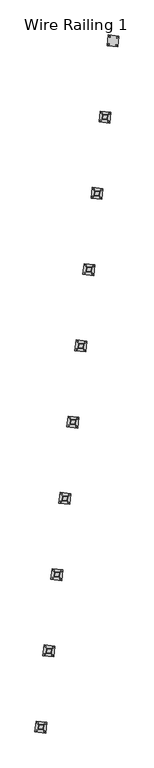
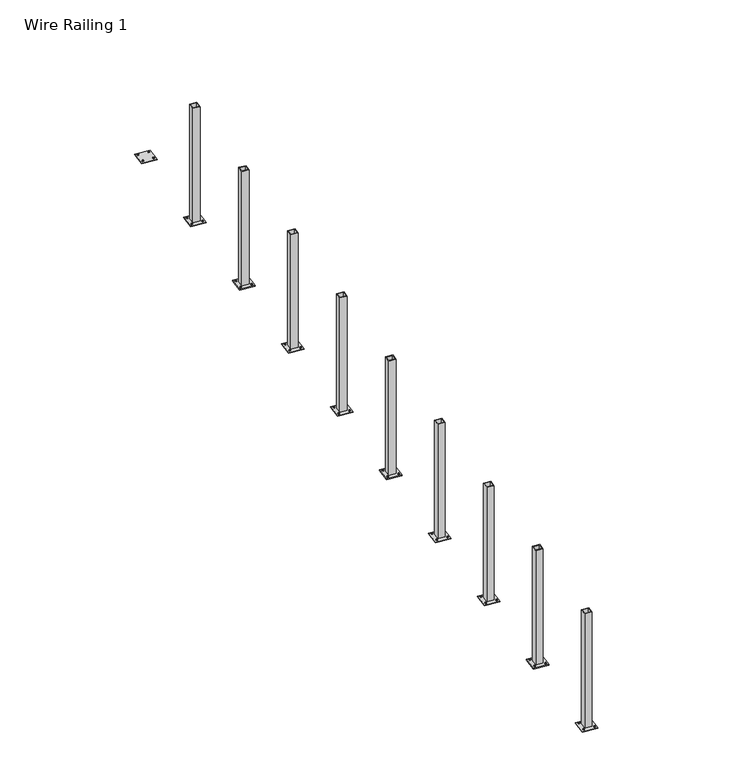
"""IFC4 building model written with IfcOpenShell, lengths in millimetres: railing geometry, Wire Railing 1."""

from ifc_helpers import new_model, si_unit, point, frame, frame_2d, origin, place, context, project, spatial, polyline, circle_curve, trimmed, segment, composite_curve, outline, extrude, source, transform, mapped, element, save


def wire_railing_1_2c713a8a(model_context):
    return source(origin(), model_context, "Body", "SweptSolid", [
        extrude(outline(composite_curve([segment(trimmed(circle_curve(frame_2d((34151.7522083, 29200.9197496)), 6.35), [point((34158.0674223, 29200.2559939))], [point((34145.4369943, 29201.5835054))], False, "CARTESIAN"), True, "CONTINUOUS"), segment(trimmed(circle_curve(frame_2d((34151.7522083, 29200.9197496)), 6.35), [point((34145.4369943, 29201.5835054))], [point((34158.0674223, 29200.2559939))], False, "CARTESIAN"), True, "CONTINUOUS")], self_intersect=False)), frame((0.0, 0.0, 266395.2), z_axis=(0.0, 0.0, 1.0), x_axis=(1.0, 0.0, 0.0)), (0.0, 0.0, 1.0), 12.7),
        extrude(outline(composite_curve([segment(trimmed(circle_curve(frame_2d((34063.3392118, 29210.21233)), 6.35), [point((34069.6544258, 29209.5485743))], [point((34057.0239978, 29210.8760857))], False, "CARTESIAN"), True, "CONTINUOUS"), segment(trimmed(circle_curve(frame_2d((34063.3392118, 29210.21233)), 6.35), [point((34057.0239978, 29210.8760857))], [point((34069.6544258, 29209.5485743))], False, "CARTESIAN"), True, "CONTINUOUS")], self_intersect=False)), frame((0.0, 0.0, 266395.2), z_axis=(0.0, 0.0, 1.0), x_axis=(1.0, 0.0, 0.0)), (0.0, 0.0, 1.0), 12.7),
        extrude(outline(composite_curve([segment(trimmed(circle_curve(frame_2d((34142.4596279, 29112.5067531)), 6.35), [point((34148.7748419, 29111.8429974))], [point((34136.1444139, 29113.1705089))], False, "CARTESIAN"), True, "CONTINUOUS"), segment(trimmed(circle_curve(frame_2d((34142.4596279, 29112.5067531)), 6.35), [point((34136.1444139, 29113.1705089))], [point((34148.7748419, 29111.8429974))], False, "CARTESIAN"), True, "CONTINUOUS")], self_intersect=False)), frame((0.0, 0.0, 266395.2), z_axis=(0.0, 0.0, 1.0), x_axis=(1.0, 0.0, 0.0)), (0.0, 0.0, 1.0), 12.7),
        extrude(outline(composite_curve([segment(trimmed(circle_curve(frame_2d((34054.0466314, 29121.7993335)), 6.35), [point((34060.3618454, 29121.1355778))], [point((34047.7314174, 29122.4630892))], False, "CARTESIAN"), True, "CONTINUOUS"), segment(trimmed(circle_curve(frame_2d((34054.0466314, 29121.7993335)), 6.35), [point((34047.7314174, 29122.4630892))], [point((34060.3618454, 29121.1355778))], False, "CARTESIAN"), True, "CONTINUOUS")], self_intersect=False)), frame((0.0, 0.0, 266395.2), z_axis=(0.0, 0.0, 1.0), x_axis=(1.0, 0.0, 0.0)), (0.0, 0.0, 1.0), 12.7),
        extrude(outline(polyline([(34046.3848369, 29231.1492393), (34172.6891176, 29217.8741245), (34159.4140028, 29091.5698438), (34033.1097221, 29104.8449586), (34046.3848369, 29231.1492393)])), frame((0.0, 0.0, 266395.2), z_axis=(0.0, 0.0, 1.0), x_axis=(1.0, 0.0, 0.0)), (0.0, 0.0, 1.0), 6.35),
        extrude(outline(polyline([(34076.054993, 29194.509648), (34136.0495263, 29188.2039684), (34129.7438467, 29128.2094351), (34069.7493134, 29134.5151147), (34076.054993, 29194.509648)]), holes=[polyline([(34081.7064512, 29187.5306782), (34076.7282832, 29140.166573), (34124.0923885, 29135.1884049), (34129.0705565, 29182.5525102), (34081.7064512, 29187.5306782)])]), frame((0.0, 0.0, 266395.2), z_axis=(0.0, 0.0, 1.0), x_axis=(1.0, 0.0, 0.0)), (0.0, 0.0, 1.0), 1047.75),
        extrude(outline(composite_curve([segment(trimmed(circle_curve(frame_2d((34245.7300141, 30095.0588447)), 6.35), [point((34252.0452281, 30094.395089))], [point((34239.4148001, 30095.7226004))], False, "CARTESIAN"), True, "CONTINUOUS"), segment(trimmed(circle_curve(frame_2d((34245.7300141, 30095.0588447)), 6.35), [point((34239.4148001, 30095.7226004))], [point((34252.0452281, 30094.395089))], False, "CARTESIAN"), True, "CONTINUOUS")], self_intersect=False)), frame((0.0, 0.0, 266395.2), z_axis=(0.0, 0.0, 1.0), x_axis=(1.0, 0.0, 0.0)), (0.0, 0.0, 1.0), 12.7),
        extrude(outline(composite_curve([segment(trimmed(circle_curve(frame_2d((34157.3170176, 30104.3514251)), 6.35), [point((34163.6322316, 30103.6876693))], [point((34151.0018036, 30105.0151808))], False, "CARTESIAN"), True, "CONTINUOUS"), segment(trimmed(circle_curve(frame_2d((34157.3170176, 30104.3514251)), 6.35), [point((34151.0018036, 30105.0151808))], [point((34163.6322316, 30103.6876693))], False, "CARTESIAN"), True, "CONTINUOUS")], self_intersect=False)), frame((0.0, 0.0, 266395.2), z_axis=(0.0, 0.0, 1.0), x_axis=(1.0, 0.0, 0.0)), (0.0, 0.0, 1.0), 12.7),
        extrude(outline(composite_curve([segment(trimmed(circle_curve(frame_2d((34236.4374337, 30006.6458482)), 6.35), [point((34242.7526478, 30005.9820925))], [point((34230.1222197, 30007.3096039))], False, "CARTESIAN"), True, "CONTINUOUS"), segment(trimmed(circle_curve(frame_2d((34236.4374337, 30006.6458482)), 6.35), [point((34230.1222197, 30007.3096039))], [point((34242.7526478, 30005.9820925))], False, "CARTESIAN"), True, "CONTINUOUS")], self_intersect=False)), frame((0.0, 0.0, 266395.2), z_axis=(0.0, 0.0, 1.0), x_axis=(1.0, 0.0, 0.0)), (0.0, 0.0, 1.0), 12.7),
        extrude(outline(composite_curve([segment(trimmed(circle_curve(frame_2d((34148.0244372, 30015.9384286)), 6.35), [point((34154.3396513, 30015.2746728))], [point((34141.7092232, 30016.6021843))], False, "CARTESIAN"), True, "CONTINUOUS"), segment(trimmed(circle_curve(frame_2d((34148.0244372, 30015.9384286)), 6.35), [point((34141.7092232, 30016.6021843))], [point((34154.3396513, 30015.2746728))], False, "CARTESIAN"), True, "CONTINUOUS")], self_intersect=False)), frame((0.0, 0.0, 266395.2), z_axis=(0.0, 0.0, 1.0), x_axis=(1.0, 0.0, 0.0)), (0.0, 0.0, 1.0), 12.7),
        extrude(outline(polyline([(34140.3626427, 30125.2883344), (34266.6669234, 30112.0132196), (34253.3918086, 29985.7089389), (34127.0875279, 29998.9840537), (34140.3626427, 30125.2883344)])), frame((0.0, 0.0, 266395.2), z_axis=(0.0, 0.0, 1.0), x_axis=(1.0, 0.0, 0.0)), (0.0, 0.0, 1.0), 6.35),
        extrude(outline(polyline([(34170.0327988, 30088.6487431), (34230.0273321, 30082.3430635), (34223.7216526, 30022.3485302), (34163.7271192, 30028.6542097), (34170.0327988, 30088.6487431)]), holes=[polyline([(34175.6842571, 30081.6697733), (34170.706089, 30034.305668), (34218.0701943, 30029.3275), (34223.0483623, 30076.6916052), (34175.6842571, 30081.6697733)])]), frame((0.0, 0.0, 266395.2), z_axis=(0.0, 0.0, 1.0), x_axis=(1.0, 0.0, 0.0)), (0.0, 0.0, 1.0), 1047.75),
        extrude(outline(composite_curve([segment(trimmed(circle_curve(frame_2d((34339.7078199, 30989.1979398)), 6.35), [point((34346.0230339, 30988.534184))], [point((34333.3926059, 30989.8616955))], False, "CARTESIAN"), True, "CONTINUOUS"), segment(trimmed(circle_curve(frame_2d((34339.7078199, 30989.1979398)), 6.35), [point((34333.3926059, 30989.8616955))], [point((34346.0230339, 30988.534184))], False, "CARTESIAN"), True, "CONTINUOUS")], self_intersect=False)), frame((0.0, 0.0, 266395.2), z_axis=(0.0, 0.0, 1.0), x_axis=(1.0, 0.0, 0.0)), (0.0, 0.0, 1.0), 12.7),
        extrude(outline(composite_curve([segment(trimmed(circle_curve(frame_2d((34251.2948234, 30998.4905202)), 6.35), [point((34257.6100375, 30997.8267644))], [point((34244.9796094, 30999.1542759))], False, "CARTESIAN"), True, "CONTINUOUS"), segment(trimmed(circle_curve(frame_2d((34251.2948234, 30998.4905202)), 6.35), [point((34244.9796094, 30999.1542759))], [point((34257.6100375, 30997.8267644))], False, "CARTESIAN"), True, "CONTINUOUS")], self_intersect=False)), frame((0.0, 0.0, 266395.2), z_axis=(0.0, 0.0, 1.0), x_axis=(1.0, 0.0, 0.0)), (0.0, 0.0, 1.0), 12.7),
        extrude(outline(composite_curve([segment(trimmed(circle_curve(frame_2d((34330.4152395, 30900.7849433)), 6.35), [point((34336.7304536, 30900.1211875))], [point((34324.1000255, 30901.448699))], False, "CARTESIAN"), True, "CONTINUOUS"), segment(trimmed(circle_curve(frame_2d((34330.4152395, 30900.7849433)), 6.35), [point((34324.1000255, 30901.448699))], [point((34336.7304536, 30900.1211875))], False, "CARTESIAN"), True, "CONTINUOUS")], self_intersect=False)), frame((0.0, 0.0, 266395.2), z_axis=(0.0, 0.0, 1.0), x_axis=(1.0, 0.0, 0.0)), (0.0, 0.0, 1.0), 12.7),
        extrude(outline(composite_curve([segment(trimmed(circle_curve(frame_2d((34242.002243, 30910.0775237)), 6.35), [point((34248.3174571, 30909.4137679))], [point((34235.687029, 30910.7412794))], False, "CARTESIAN"), True, "CONTINUOUS"), segment(trimmed(circle_curve(frame_2d((34242.002243, 30910.0775237)), 6.35), [point((34235.687029, 30910.7412794))], [point((34248.3174571, 30909.4137679))], False, "CARTESIAN"), True, "CONTINUOUS")], self_intersect=False)), frame((0.0, 0.0, 266395.2), z_axis=(0.0, 0.0, 1.0), x_axis=(1.0, 0.0, 0.0)), (0.0, 0.0, 1.0), 12.7),
        extrude(outline(polyline([(34234.3404485, 31019.4274295), (34360.6447292, 31006.1523147), (34347.3696144, 30879.848034), (34221.0653337, 30893.1231488), (34234.3404485, 31019.4274295)])), frame((0.0, 0.0, 266395.2), z_axis=(0.0, 0.0, 1.0), x_axis=(1.0, 0.0, 0.0)), (0.0, 0.0, 1.0), 6.35),
        extrude(outline(polyline([(34264.0106046, 30982.7878382), (34324.0051379, 30976.4821586), (34317.6994584, 30916.4876253), (34257.704925, 30922.7933048), (34264.0106046, 30982.7878382)]), holes=[polyline([(34269.6620629, 30975.8088684), (34264.6838948, 30928.4447631), (34312.0480001, 30923.4665951), (34317.0261681, 30970.8307003), (34269.6620629, 30975.8088684)])]), frame((0.0, 0.0, 266395.2), z_axis=(0.0, 0.0, 1.0), x_axis=(1.0, 0.0, 0.0)), (0.0, 0.0, 1.0), 1047.75),
        extrude(outline(composite_curve([segment(trimmed(circle_curve(frame_2d((34433.6856257, 31883.3370349)), 6.35), [point((34440.0008398, 31882.6732791))], [point((34427.3704117, 31884.0007906))], False, "CARTESIAN"), True, "CONTINUOUS"), segment(trimmed(circle_curve(frame_2d((34433.6856257, 31883.3370349)), 6.35), [point((34427.3704117, 31884.0007906))], [point((34440.0008398, 31882.6732791))], False, "CARTESIAN"), True, "CONTINUOUS")], self_intersect=False)), frame((0.0, 0.0, 266395.2), z_axis=(0.0, 0.0, 1.0), x_axis=(1.0, 0.0, 0.0)), (0.0, 0.0, 1.0), 12.7),
        extrude(outline(composite_curve([segment(trimmed(circle_curve(frame_2d((34345.2726292, 31892.6296153)), 6.35), [point((34351.5878433, 31891.9658595))], [point((34338.9574152, 31893.293371))], False, "CARTESIAN"), True, "CONTINUOUS"), segment(trimmed(circle_curve(frame_2d((34345.2726292, 31892.6296153)), 6.35), [point((34338.9574152, 31893.293371))], [point((34351.5878433, 31891.9658595))], False, "CARTESIAN"), True, "CONTINUOUS")], self_intersect=False)), frame((0.0, 0.0, 266395.2), z_axis=(0.0, 0.0, 1.0), x_axis=(1.0, 0.0, 0.0)), (0.0, 0.0, 1.0), 12.7),
        extrude(outline(composite_curve([segment(trimmed(circle_curve(frame_2d((34424.3930453, 31794.9240384)), 6.35), [point((34430.7082594, 31794.2602826))], [point((34418.0778313, 31795.5877941))], False, "CARTESIAN"), True, "CONTINUOUS"), segment(trimmed(circle_curve(frame_2d((34424.3930453, 31794.9240384)), 6.35), [point((34418.0778313, 31795.5877941))], [point((34430.7082594, 31794.2602826))], False, "CARTESIAN"), True, "CONTINUOUS")], self_intersect=False)), frame((0.0, 0.0, 266395.2), z_axis=(0.0, 0.0, 1.0), x_axis=(1.0, 0.0, 0.0)), (0.0, 0.0, 1.0), 12.7),
        extrude(outline(composite_curve([segment(trimmed(circle_curve(frame_2d((34335.9800488, 31804.2166188)), 6.35), [point((34342.2952629, 31803.552863))], [point((34329.6648348, 31804.8803745))], False, "CARTESIAN"), True, "CONTINUOUS"), segment(trimmed(circle_curve(frame_2d((34335.9800488, 31804.2166188)), 6.35), [point((34329.6648348, 31804.8803745))], [point((34342.2952629, 31803.552863))], False, "CARTESIAN"), True, "CONTINUOUS")], self_intersect=False)), frame((0.0, 0.0, 266395.2), z_axis=(0.0, 0.0, 1.0), x_axis=(1.0, 0.0, 0.0)), (0.0, 0.0, 1.0), 12.7),
        extrude(outline(polyline([(34328.3182543, 31913.5665246), (34454.6225351, 31900.2914098), (34441.3474202, 31773.987129), (34315.0431395, 31787.2622439), (34328.3182543, 31913.5665246)])), frame((0.0, 0.0, 266395.2), z_axis=(0.0, 0.0, 1.0), x_axis=(1.0, 0.0, 0.0)), (0.0, 0.0, 1.0), 6.35),
        extrude(outline(polyline([(34357.9884104, 31876.9269333), (34417.9829437, 31870.6212537), (34411.6772642, 31810.6267204), (34351.6827308, 31816.9323999), (34357.9884104, 31876.9269333)]), holes=[polyline([(34363.6398687, 31869.9479635), (34358.6617006, 31822.5838582), (34406.0258059, 31817.6056902), (34411.0039739, 31864.9697954), (34363.6398687, 31869.9479635)])]), frame((0.0, 0.0, 266395.2), z_axis=(0.0, 0.0, 1.0), x_axis=(1.0, 0.0, 0.0)), (0.0, 0.0, 1.0), 1047.75),
        extrude(outline(composite_curve([segment(trimmed(circle_curve(frame_2d((34527.6634315, 32777.47613)), 6.35), [point((34533.9786456, 32776.8123742))], [point((34521.3482175, 32778.1398857))], False, "CARTESIAN"), True, "CONTINUOUS"), segment(trimmed(circle_curve(frame_2d((34527.6634315, 32777.47613)), 6.35), [point((34521.3482175, 32778.1398857))], [point((34533.9786456, 32776.8123742))], False, "CARTESIAN"), True, "CONTINUOUS")], self_intersect=False)), frame((0.0, 0.0, 266395.2), z_axis=(0.0, 0.0, 1.0), x_axis=(1.0, 0.0, 0.0)), (0.0, 0.0, 1.0), 12.7),
        extrude(outline(composite_curve([segment(trimmed(circle_curve(frame_2d((34439.250435, 32786.7687104)), 6.35), [point((34445.5656491, 32786.1049546))], [point((34432.935221, 32787.4324661))], False, "CARTESIAN"), True, "CONTINUOUS"), segment(trimmed(circle_curve(frame_2d((34439.250435, 32786.7687104)), 6.35), [point((34432.935221, 32787.4324661))], [point((34445.5656491, 32786.1049546))], False, "CARTESIAN"), True, "CONTINUOUS")], self_intersect=False)), frame((0.0, 0.0, 266395.2), z_axis=(0.0, 0.0, 1.0), x_axis=(1.0, 0.0, 0.0)), (0.0, 0.0, 1.0), 12.7),
        extrude(outline(composite_curve([segment(trimmed(circle_curve(frame_2d((34518.3708511, 32689.0631335)), 6.35), [point((34524.6860652, 32688.3993777))], [point((34512.0556371, 32689.7268892))], False, "CARTESIAN"), True, "CONTINUOUS"), segment(trimmed(circle_curve(frame_2d((34518.3708511, 32689.0631335)), 6.35), [point((34512.0556371, 32689.7268892))], [point((34524.6860652, 32688.3993777))], False, "CARTESIAN"), True, "CONTINUOUS")], self_intersect=False)), frame((0.0, 0.0, 266395.2), z_axis=(0.0, 0.0, 1.0), x_axis=(1.0, 0.0, 0.0)), (0.0, 0.0, 1.0), 12.7),
        extrude(outline(composite_curve([segment(trimmed(circle_curve(frame_2d((34429.9578547, 32698.3557139)), 6.35), [point((34436.2730687, 32697.6919581))], [point((34423.6426406, 32699.0194696))], False, "CARTESIAN"), True, "CONTINUOUS"), segment(trimmed(circle_curve(frame_2d((34429.9578547, 32698.3557139)), 6.35), [point((34423.6426406, 32699.0194696))], [point((34436.2730687, 32697.6919581))], False, "CARTESIAN"), True, "CONTINUOUS")], self_intersect=False)), frame((0.0, 0.0, 266395.2), z_axis=(0.0, 0.0, 1.0), x_axis=(1.0, 0.0, 0.0)), (0.0, 0.0, 1.0), 12.7),
        extrude(outline(polyline([(34422.2960602, 32807.7056197), (34548.6003409, 32794.4305048), (34535.325226, 32668.1262241), (34409.0209453, 32681.401339), (34422.2960602, 32807.7056197)])), frame((0.0, 0.0, 266395.2), z_axis=(0.0, 0.0, 1.0), x_axis=(1.0, 0.0, 0.0)), (0.0, 0.0, 1.0), 6.35),
        extrude(outline(polyline([(34451.9662162, 32771.0660284), (34511.9607495, 32764.7603488), (34505.65507, 32704.7658155), (34445.6605367, 32711.071495), (34451.9662162, 32771.0660284)]), holes=[polyline([(34457.6176745, 32764.0870586), (34452.6395064, 32716.7229533), (34500.0036117, 32711.7447852), (34504.9817798, 32759.1088905), (34457.6176745, 32764.0870586)])]), frame((0.0, 0.0, 266395.2), z_axis=(0.0, 0.0, 1.0), x_axis=(1.0, 0.0, 0.0)), (0.0, 0.0, 1.0), 1047.75),
        extrude(outline(composite_curve([segment(trimmed(circle_curve(frame_2d((34621.6412373, 33671.6152251)), 6.35), [point((34627.9564514, 33670.9514693))], [point((34615.3260233, 33672.2789808))], False, "CARTESIAN"), True, "CONTINUOUS"), segment(trimmed(circle_curve(frame_2d((34621.6412373, 33671.6152251)), 6.35), [point((34615.3260233, 33672.2789808))], [point((34627.9564514, 33670.9514693))], False, "CARTESIAN"), True, "CONTINUOUS")], self_intersect=False)), frame((0.0, 0.0, 266395.2), z_axis=(0.0, 0.0, 1.0), x_axis=(1.0, 0.0, 0.0)), (0.0, 0.0, 1.0), 12.7),
        extrude(outline(composite_curve([segment(trimmed(circle_curve(frame_2d((34533.2282408, 33680.9078054)), 6.35), [point((34539.5434549, 33680.2440497))], [point((34526.9130268, 33681.5715612))], False, "CARTESIAN"), True, "CONTINUOUS"), segment(trimmed(circle_curve(frame_2d((34533.2282408, 33680.9078054)), 6.35), [point((34526.9130268, 33681.5715612))], [point((34539.5434549, 33680.2440497))], False, "CARTESIAN"), True, "CONTINUOUS")], self_intersect=False)), frame((0.0, 0.0, 266395.2), z_axis=(0.0, 0.0, 1.0), x_axis=(1.0, 0.0, 0.0)), (0.0, 0.0, 1.0), 12.7),
        extrude(outline(composite_curve([segment(trimmed(circle_curve(frame_2d((34612.348657, 33583.2022286)), 6.35), [point((34618.663871, 33582.5384728))], [point((34606.0334429, 33583.8659843))], False, "CARTESIAN"), True, "CONTINUOUS"), segment(trimmed(circle_curve(frame_2d((34612.348657, 33583.2022286)), 6.35), [point((34606.0334429, 33583.8659843))], [point((34618.663871, 33582.5384728))], False, "CARTESIAN"), True, "CONTINUOUS")], self_intersect=False)), frame((0.0, 0.0, 266395.2), z_axis=(0.0, 0.0, 1.0), x_axis=(1.0, 0.0, 0.0)), (0.0, 0.0, 1.0), 12.7),
        extrude(outline(composite_curve([segment(trimmed(circle_curve(frame_2d((34523.9356605, 33592.4948089)), 6.35), [point((34530.2508745, 33591.8310532))], [point((34517.6204464, 33593.1585647))], False, "CARTESIAN"), True, "CONTINUOUS"), segment(trimmed(circle_curve(frame_2d((34523.9356605, 33592.4948089)), 6.35), [point((34517.6204464, 33593.1585647))], [point((34530.2508745, 33591.8310532))], False, "CARTESIAN"), True, "CONTINUOUS")], self_intersect=False)), frame((0.0, 0.0, 266395.2), z_axis=(0.0, 0.0, 1.0), x_axis=(1.0, 0.0, 0.0)), (0.0, 0.0, 1.0), 12.7),
        extrude(outline(polyline([(34516.273866, 33701.8447148), (34642.5781467, 33688.5695999), (34629.3030318, 33562.2653192), (34502.9987511, 33575.5404341), (34516.273866, 33701.8447148)])), frame((0.0, 0.0, 266395.2), z_axis=(0.0, 0.0, 1.0), x_axis=(1.0, 0.0, 0.0)), (0.0, 0.0, 1.0), 6.35),
        extrude(outline(polyline([(34545.944022, 33665.2051234), (34605.9385553, 33658.8994439), (34599.6328758, 33598.9049106), (34539.6383425, 33605.2105901), (34545.944022, 33665.2051234)]), holes=[polyline([(34551.5954803, 33658.2261537), (34546.6173122, 33610.8620484), (34593.9814175, 33605.8838803), (34598.9595856, 33653.2479856), (34551.5954803, 33658.2261537)])]), frame((0.0, 0.0, 266395.2), z_axis=(0.0, 0.0, 1.0), x_axis=(1.0, 0.0, 0.0)), (0.0, 0.0, 1.0), 1047.75),
        extrude(outline(composite_curve([segment(trimmed(circle_curve(frame_2d((34715.6190432, 34565.7543201)), 6.35), [point((34721.9342572, 34565.0905644))], [point((34709.3038291, 34566.4180759))], False, "CARTESIAN"), True, "CONTINUOUS"), segment(trimmed(circle_curve(frame_2d((34715.6190432, 34565.7543201)), 6.35), [point((34709.3038291, 34566.4180759))], [point((34721.9342572, 34565.0905644))], False, "CARTESIAN"), True, "CONTINUOUS")], self_intersect=False)), frame((0.0, 0.0, 266395.2), z_axis=(0.0, 0.0, 1.0), x_axis=(1.0, 0.0, 0.0)), (0.0, 0.0, 1.0), 12.7),
        extrude(outline(composite_curve([segment(trimmed(circle_curve(frame_2d((34627.2060467, 34575.0469005)), 6.35), [point((34633.5212607, 34574.3831448))], [point((34620.8908326, 34575.7106563))], False, "CARTESIAN"), True, "CONTINUOUS"), segment(trimmed(circle_curve(frame_2d((34627.2060467, 34575.0469005)), 6.35), [point((34620.8908326, 34575.7106563))], [point((34633.5212607, 34574.3831448))], False, "CARTESIAN"), True, "CONTINUOUS")], self_intersect=False)), frame((0.0, 0.0, 266395.2), z_axis=(0.0, 0.0, 1.0), x_axis=(1.0, 0.0, 0.0)), (0.0, 0.0, 1.0), 12.7),
        extrude(outline(composite_curve([segment(trimmed(circle_curve(frame_2d((34706.3264628, 34477.3413236)), 6.35), [point((34712.6416768, 34476.6775679))], [point((34700.0112487, 34478.0050794))], False, "CARTESIAN"), True, "CONTINUOUS"), segment(trimmed(circle_curve(frame_2d((34706.3264628, 34477.3413236)), 6.35), [point((34700.0112487, 34478.0050794))], [point((34712.6416768, 34476.6775679))], False, "CARTESIAN"), True, "CONTINUOUS")], self_intersect=False)), frame((0.0, 0.0, 266395.2), z_axis=(0.0, 0.0, 1.0), x_axis=(1.0, 0.0, 0.0)), (0.0, 0.0, 1.0), 12.7),
        extrude(outline(composite_curve([segment(trimmed(circle_curve(frame_2d((34617.9134663, 34486.633904)), 6.35), [point((34624.2286803, 34485.9701483))], [point((34611.5982522, 34487.2976598))], False, "CARTESIAN"), True, "CONTINUOUS"), segment(trimmed(circle_curve(frame_2d((34617.9134663, 34486.633904)), 6.35), [point((34611.5982522, 34487.2976598))], [point((34624.2286803, 34485.9701483))], False, "CARTESIAN"), True, "CONTINUOUS")], self_intersect=False)), frame((0.0, 0.0, 266395.2), z_axis=(0.0, 0.0, 1.0), x_axis=(1.0, 0.0, 0.0)), (0.0, 0.0, 1.0), 12.7),
        extrude(outline(polyline([(34610.2516718, 34595.9838099), (34736.5559525, 34582.708695), (34723.2808377, 34456.4044143), (34596.9765569, 34469.6795292), (34610.2516718, 34595.9838099)])), frame((0.0, 0.0, 266395.2), z_axis=(0.0, 0.0, 1.0), x_axis=(1.0, 0.0, 0.0)), (0.0, 0.0, 1.0), 6.35),
        extrude(outline(polyline([(34639.9218278, 34559.3442185), (34699.9163612, 34553.038539), (34693.6106816, 34493.0440056), (34633.6161483, 34499.3496852), (34639.9218278, 34559.3442185)]), holes=[polyline([(34645.5732861, 34552.3652488), (34640.595118, 34505.0011435), (34687.9592233, 34500.0229754), (34692.9373914, 34547.3870807), (34645.5732861, 34552.3652488)])]), frame((0.0, 0.0, 266395.2), z_axis=(0.0, 0.0, 1.0), x_axis=(1.0, 0.0, 0.0)), (0.0, 0.0, 1.0), 1047.75),
        extrude(outline(composite_curve([segment(trimmed(circle_curve(frame_2d((34809.596849, 35459.8934152)), 6.35), [point((34815.912063, 35459.2296595))], [point((34803.2816349, 35460.557171))], False, "CARTESIAN"), True, "CONTINUOUS"), segment(trimmed(circle_curve(frame_2d((34809.596849, 35459.8934152)), 6.35), [point((34803.2816349, 35460.557171))], [point((34815.912063, 35459.2296595))], False, "CARTESIAN"), True, "CONTINUOUS")], self_intersect=False)), frame((0.0, 0.0, 266395.2), z_axis=(0.0, 0.0, 1.0), x_axis=(1.0, 0.0, 0.0)), (0.0, 0.0, 1.0), 12.7),
        extrude(outline(composite_curve([segment(trimmed(circle_curve(frame_2d((34721.1838525, 35469.1859956)), 6.35), [point((34727.4990665, 35468.5222399))], [point((34714.8686384, 35469.8497514))], False, "CARTESIAN"), True, "CONTINUOUS"), segment(trimmed(circle_curve(frame_2d((34721.1838525, 35469.1859956)), 6.35), [point((34714.8686384, 35469.8497514))], [point((34727.4990665, 35468.5222399))], False, "CARTESIAN"), True, "CONTINUOUS")], self_intersect=False)), frame((0.0, 0.0, 266395.2), z_axis=(0.0, 0.0, 1.0), x_axis=(1.0, 0.0, 0.0)), (0.0, 0.0, 1.0), 12.7),
        extrude(outline(composite_curve([segment(trimmed(circle_curve(frame_2d((34800.3042686, 35371.4804187)), 6.35), [point((34806.6194826, 35370.816663))], [point((34793.9890545, 35372.1441745))], False, "CARTESIAN"), True, "CONTINUOUS"), segment(trimmed(circle_curve(frame_2d((34800.3042686, 35371.4804187)), 6.35), [point((34793.9890545, 35372.1441745))], [point((34806.6194826, 35370.816663))], False, "CARTESIAN"), True, "CONTINUOUS")], self_intersect=False)), frame((0.0, 0.0, 266395.2), z_axis=(0.0, 0.0, 1.0), x_axis=(1.0, 0.0, 0.0)), (0.0, 0.0, 1.0), 12.7),
        extrude(outline(composite_curve([segment(trimmed(circle_curve(frame_2d((34711.8912721, 35380.7729991)), 6.35), [point((34718.2064861, 35380.1092434))], [point((34705.576058, 35381.4367549))], False, "CARTESIAN"), True, "CONTINUOUS"), segment(trimmed(circle_curve(frame_2d((34711.8912721, 35380.7729991)), 6.35), [point((34705.576058, 35381.4367549))], [point((34718.2064861, 35380.1092434))], False, "CARTESIAN"), True, "CONTINUOUS")], self_intersect=False)), frame((0.0, 0.0, 266395.2), z_axis=(0.0, 0.0, 1.0), x_axis=(1.0, 0.0, 0.0)), (0.0, 0.0, 1.0), 12.7),
        extrude(outline(polyline([(34704.2294776, 35490.122905), (34830.5337583, 35476.8477901), (34817.2586435, 35350.5435094), (34690.9543628, 35363.8186242), (34704.2294776, 35490.122905)])), frame((0.0, 0.0, 266395.2), z_axis=(0.0, 0.0, 1.0), x_axis=(1.0, 0.0, 0.0)), (0.0, 0.0, 1.0), 6.35),
        extrude(outline(polyline([(34733.8996336, 35453.4833136), (34793.894167, 35447.1776341), (34787.5884874, 35387.1831007), (34727.5939541, 35393.4887803), (34733.8996336, 35453.4833136)]), holes=[polyline([(34739.5510919, 35446.5043438), (34734.5729239, 35399.1402386), (34781.9370291, 35394.1620705), (34786.9151972, 35441.5261758), (34739.5510919, 35446.5043438)])]), frame((0.0, 0.0, 266395.2), z_axis=(0.0, 0.0, 1.0), x_axis=(1.0, 0.0, 0.0)), (0.0, 0.0, 1.0), 1047.75),
        extrude(outline(composite_curve([segment(trimmed(circle_curve(frame_2d((34903.5746548, 36354.0325103)), 6.35), [point((34909.8898688, 36353.3687546))], [point((34897.2594407, 36354.6962661))], False, "CARTESIAN"), True, "CONTINUOUS"), segment(trimmed(circle_curve(frame_2d((34903.5746548, 36354.0325103)), 6.35), [point((34897.2594407, 36354.6962661))], [point((34909.8898688, 36353.3687546))], False, "CARTESIAN"), True, "CONTINUOUS")], self_intersect=False)), frame((0.0, 0.0, 266395.2), z_axis=(0.0, 0.0, 1.0), x_axis=(1.0, 0.0, 0.0)), (0.0, 0.0, 1.0), 12.7),
        extrude(outline(composite_curve([segment(trimmed(circle_curve(frame_2d((34815.1616583, 36363.3250907)), 6.35), [point((34821.4768723, 36362.661335))], [point((34808.8464442, 36363.9888465))], False, "CARTESIAN"), True, "CONTINUOUS"), segment(trimmed(circle_curve(frame_2d((34815.1616583, 36363.3250907)), 6.35), [point((34808.8464442, 36363.9888465))], [point((34821.4768723, 36362.661335))], False, "CARTESIAN"), True, "CONTINUOUS")], self_intersect=False)), frame((0.0, 0.0, 266395.2), z_axis=(0.0, 0.0, 1.0), x_axis=(1.0, 0.0, 0.0)), (0.0, 0.0, 1.0), 12.7),
        extrude(outline(composite_curve([segment(trimmed(circle_curve(frame_2d((34894.2820744, 36265.6195138)), 6.35), [point((34900.5972884, 36264.9557581))], [point((34887.9668604, 36266.2832696))], False, "CARTESIAN"), True, "CONTINUOUS"), segment(trimmed(circle_curve(frame_2d((34894.2820744, 36265.6195138)), 6.35), [point((34887.9668604, 36266.2832696))], [point((34900.5972884, 36264.9557581))], False, "CARTESIAN"), True, "CONTINUOUS")], self_intersect=False)), frame((0.0, 0.0, 266395.2), z_axis=(0.0, 0.0, 1.0), x_axis=(1.0, 0.0, 0.0)), (0.0, 0.0, 1.0), 12.7),
        extrude(outline(composite_curve([segment(trimmed(circle_curve(frame_2d((34805.8690779, 36274.9120942)), 6.35), [point((34812.1842919, 36274.2483385))], [point((34799.5538639, 36275.57585))], False, "CARTESIAN"), True, "CONTINUOUS"), segment(trimmed(circle_curve(frame_2d((34805.8690779, 36274.9120942)), 6.35), [point((34799.5538639, 36275.57585))], [point((34812.1842919, 36274.2483385))], False, "CARTESIAN"), True, "CONTINUOUS")], self_intersect=False)), frame((0.0, 0.0, 266395.2), z_axis=(0.0, 0.0, 1.0), x_axis=(1.0, 0.0, 0.0)), (0.0, 0.0, 1.0), 12.7),
        extrude(outline(polyline([(34798.2072834, 36384.262), (34924.5115641, 36370.9868852), (34911.2364493, 36244.6826045), (34784.9321686, 36257.9577193), (34798.2072834, 36384.262)])), frame((0.0, 0.0, 266395.2), z_axis=(0.0, 0.0, 1.0), x_axis=(1.0, 0.0, 0.0)), (0.0, 0.0, 1.0), 6.35),
        extrude(outline(polyline([(34827.8774394, 36347.6224087), (34887.8719728, 36341.3167292), (34881.5662932, 36281.3221958), (34821.5717599, 36287.6278754), (34827.8774394, 36347.6224087)]), holes=[polyline([(34833.5288977, 36340.6434389), (34828.5507297, 36293.2793337), (34875.9148349, 36288.3011656), (34880.893003, 36335.6652709), (34833.5288977, 36340.6434389)])]), frame((0.0, 0.0, 266395.2), z_axis=(0.0, 0.0, 1.0), x_axis=(1.0, 0.0, 0.0)), (0.0, 0.0, 1.0), 1047.75),
        extrude(outline(composite_curve([segment(trimmed(circle_curve(frame_2d((34997.5524606, 37248.1716054)), 6.35), [point((35003.8676746, 37247.5078497))], [point((34991.2372466, 37248.8353612))], False, "CARTESIAN"), True, "CONTINUOUS"), segment(trimmed(circle_curve(frame_2d((34997.5524606, 37248.1716054)), 6.35), [point((34991.2372466, 37248.8353612))], [point((35003.8676746, 37247.5078497))], False, "CARTESIAN"), True, "CONTINUOUS")], self_intersect=False)), frame((0.0, 0.0, 266395.2), z_axis=(0.0, 0.0, 1.0), x_axis=(1.0, 0.0, 0.0)), (0.0, 0.0, 1.0), 12.7),
        extrude(outline(composite_curve([segment(trimmed(circle_curve(frame_2d((34909.1394641, 37257.4641858)), 6.35), [point((34915.4546781, 37256.8004301))], [point((34902.8242501, 37258.1279415))], False, "CARTESIAN"), True, "CONTINUOUS"), segment(trimmed(circle_curve(frame_2d((34909.1394641, 37257.4641858)), 6.35), [point((34902.8242501, 37258.1279415))], [point((34915.4546781, 37256.8004301))], False, "CARTESIAN"), True, "CONTINUOUS")], self_intersect=False)), frame((0.0, 0.0, 266395.2), z_axis=(0.0, 0.0, 1.0), x_axis=(1.0, 0.0, 0.0)), (0.0, 0.0, 1.0), 12.7),
        extrude(outline(composite_curve([segment(trimmed(circle_curve(frame_2d((34988.2598802, 37159.7586089)), 6.35), [point((34994.5750942, 37159.0948532))], [point((34981.9446662, 37160.4223647))], False, "CARTESIAN"), True, "CONTINUOUS"), segment(trimmed(circle_curve(frame_2d((34988.2598802, 37159.7586089)), 6.35), [point((34981.9446662, 37160.4223647))], [point((34994.5750942, 37159.0948532))], False, "CARTESIAN"), True, "CONTINUOUS")], self_intersect=False)), frame((0.0, 0.0, 266395.2), z_axis=(0.0, 0.0, 1.0), x_axis=(1.0, 0.0, 0.0)), (0.0, 0.0, 1.0), 12.7),
        extrude(outline(composite_curve([segment(trimmed(circle_curve(frame_2d((34899.8468837, 37169.0511893)), 6.35), [point((34906.1620977, 37168.3874336))], [point((34893.5316697, 37169.714945))], False, "CARTESIAN"), True, "CONTINUOUS"), segment(trimmed(circle_curve(frame_2d((34899.8468837, 37169.0511893)), 6.35), [point((34893.5316697, 37169.714945))], [point((34906.1620977, 37168.3874336))], False, "CARTESIAN"), True, "CONTINUOUS")], self_intersect=False)), frame((0.0, 0.0, 266395.2), z_axis=(0.0, 0.0, 1.0), x_axis=(1.0, 0.0, 0.0)), (0.0, 0.0, 1.0), 12.7),
        extrude(outline(polyline([(34892.1850892, 37278.4010951), (35018.4893699, 37265.1259803), (35005.2142551, 37138.8216996), (34878.9099744, 37152.0968144), (34892.1850892, 37278.4010951)])), frame((0.0, 0.0, 266395.2), z_axis=(0.0, 0.0, 1.0), x_axis=(1.0, 0.0, 0.0)), (0.0, 0.0, 1.0), 6.35),
    ])


if __name__ == "__main__":
    model = new_model("IFC4")
    model_context = context("Model", 3, world=origin())
    ifc_project = project(units=[si_unit("LENGTHUNIT", "METRE", prefix="MILLI")], contexts=[model_context])
    site = spatial("IfcSite", under=ifc_project)
    building = spatial("IfcBuilding", under=site)
    placement = place(None, origin())
    wire_railing_1_shape = wire_railing_1_2c713a8a(model_context)
    element("IfcRailing", 1, ObjectType="Wire Railing 1", at=placement, inside=building, context=model_context, shape_type="MappedRepresentation", body=[
        mapped(wire_railing_1_shape, transform((0.0, 0.0, 0.0), x_axis=(1.0, 0.0, 0.0), y_axis=(0.0, 1.0, 0.0), z_axis=(0.0, 0.0, 1.0))),
    ])
    save(model, "model.ifc")

# Revit data of these elements
# Element 1 (IfcRailing, "Wire Railing 1")
#   Materials on its faces: "WIRE RAILING"
# Materials
#   "WIRE RAILING": class "Metal", colour RGB 244 244 244, transparency 0, Manufacturer = "Kawneer", URL = "http://www.kawneer.com/kawneer/north_america/en/home.asp", Cost = 0
